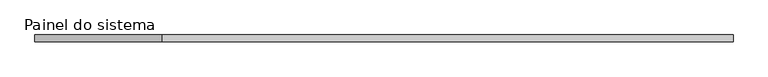
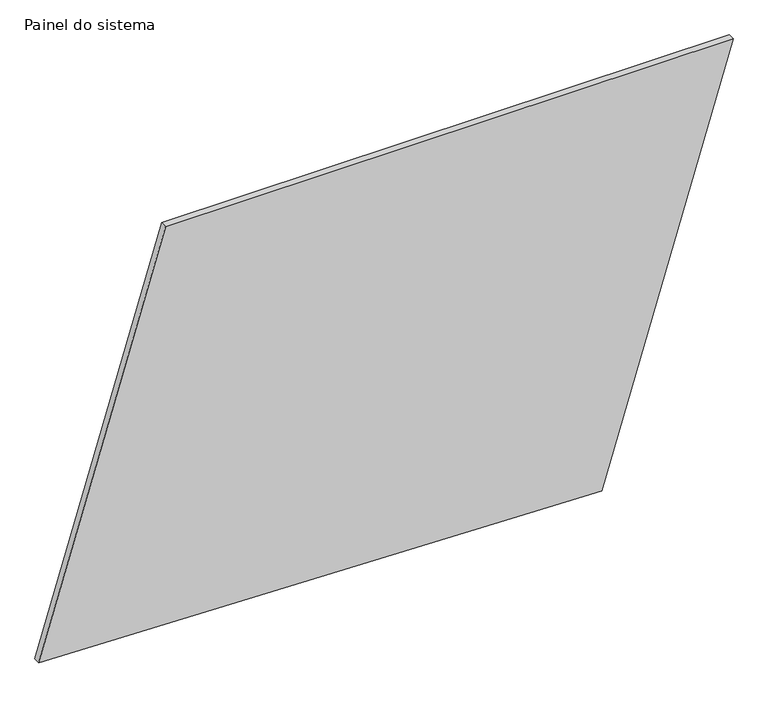
"""IFC4 building model written with IfcOpenShell, lengths in millimetres: plate geometry, Painel do sistema : Envidraçado."""

from ifc_helpers import new_model, si_unit, frame, origin, place, context, project, spatial, polyline, outline, extrude, source, transform, mapped, element, save


def painel_do_sistema_206ab684(model_context):
    return source(origin(), model_context, "Body", "SweptSolid", [
        extrude(outline(polyline([(57.0017304, -1318.2869385), (0.0, 819.4037753), (1641.1151917, 1318.2869385), (1641.1151917, -836.7317506), (57.0017304, -1318.2869385)])), frame((0.0, 24.5, 0.0), z_axis=(0.0, 1.0, 0.0), x_axis=(0.0, 0.0, 1.0)), (0.0, 0.0, 1.0), 25.0),
    ])


if __name__ == "__main__":
    model = new_model("IFC4")
    model_context = context("Model", 3, world=origin())
    ifc_project = project(units=[si_unit("LENGTHUNIT", "METRE", prefix="MILLI")], contexts=[model_context])
    site = spatial("IfcSite", under=ifc_project)
    building = spatial("IfcBuilding", under=site)
    placement = place(None, origin())
    painel_do_sistema_shape = painel_do_sistema_206ab684(model_context)
    element("IfcPlate", 1, ObjectType="Painel do sistema : Envidraçado", at=placement, inside=building, context=model_context, shape_type="MappedRepresentation", body=[
        mapped(painel_do_sistema_shape, transform((0.0, 0.0, 0.0), x_axis=(1.0, 0.0, 0.0), y_axis=(0.0, 1.0, 0.0), z_axis=(0.0, 0.0, 1.0))),
    ])
    save(model, "model.ifc")

# Revit data of these elements
# Type "Painel do sistema : Envidraçado"
#   Construction Type Id = "GSP4R"
#   Analytic Construction = "Vidraça única Pilkington 1/8 pol"
#   Visual Light Transmittance = 0.9
#   Solar Heat Gain Coefficient = 0.86
#   Heat Transfer Coefficient (U) = 6.7069 W/(m²·K)
# Element 1 (IfcPlate, "Painel do sistema : Envidraçado")
#   Materials on its faces: "Vidro"
# Materials
#   "Vidro": class "Vidro", colour RGB 0 128 192, transparency 0.9, Description = "Vidro de sílica", Cost = 0
